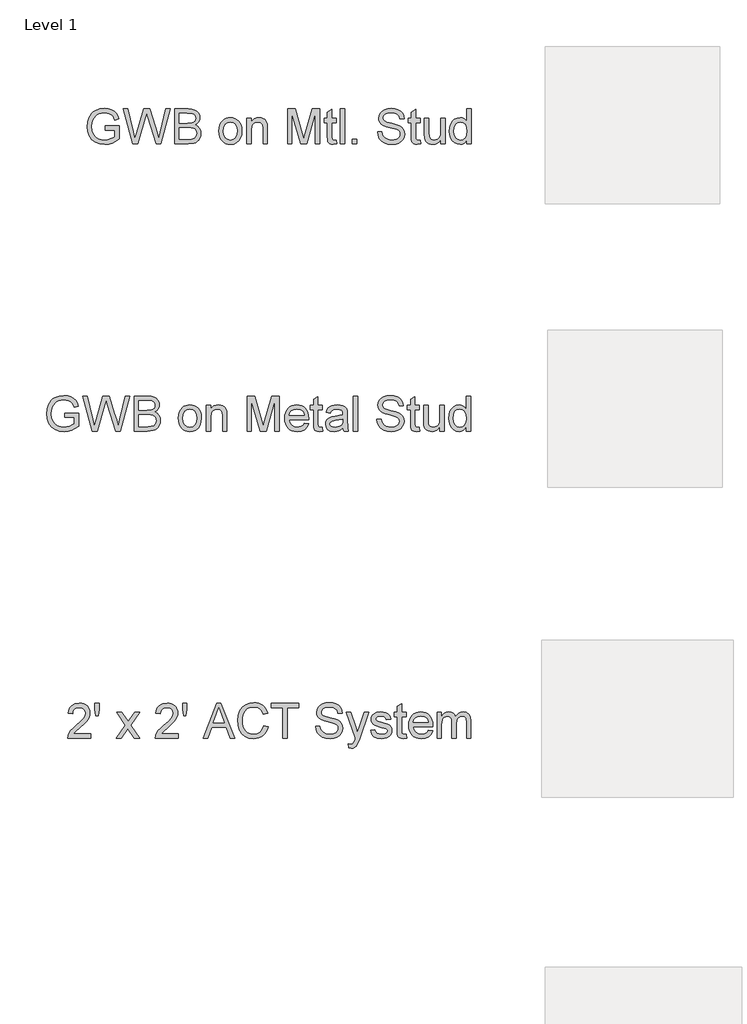
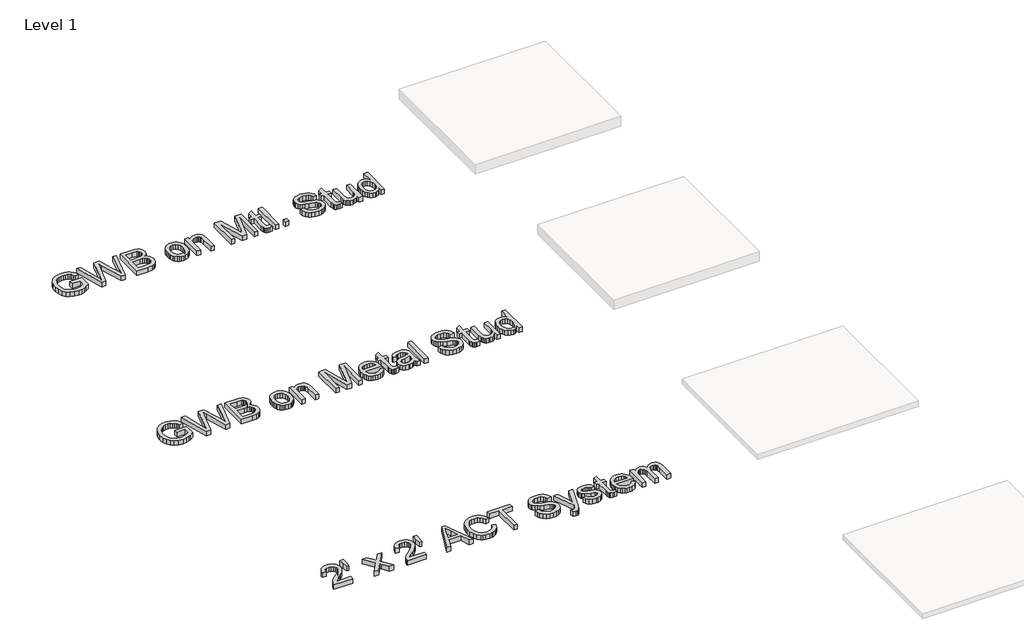
# One storey, part 11 of 42: 3 proxies.
"""IFC4 building model written with IfcOpenShell, lengths in millimetres."""

from ifc_helpers import new_model, si_unit, origin, origin_with_axes, place, context, project, spatial, polyline, outline, extrude, element, save

model = new_model("IFC4")

# Units and contexts
model_context = context("Model", 3, world=origin())
ifc_project = project(units=[si_unit("LENGTHUNIT", "METRE", prefix="MILLI")], contexts=[model_context])

# Site, building, storey
site = spatial("IfcSite", under=ifc_project)
building = spatial("IfcBuilding", under=site)
storey = spatial("IfcBuildingStorey", under=building, Name="Level 1", Elevation=0.0)

# Proxies
placement = place(None, origin())
element("IfcBuildingElementProxy", 1, Name="8\" Arial", ObjectType="8\" Arial", at=placement, inside=storey, context=model_context, shape_type="SweptSolid", body=[
    extrude(outline(polyline([(6999.2760884, -8581.268146), (6999.2760884, -8543.1972592), (7123.0064704, -8543.1972592), (7123.0064704, -8657.0381335), (7092.9382773, -8677.9510962), (7061.92203, -8692.9526615), (7030.0320856, -8701.9870613), (6997.3428012, -8704.998528), (6954.633884, -8700.2117832), (6916.0332022, -8685.8515488), (6883.9666594, -8662.4197359), (6860.8601593, -8630.4182557), (6846.8903002, -8592.0313508), (6842.2336805, -8549.4432641), (6846.8717109, -8506.5484539), (6860.7858021, -8466.6465211), (6883.3996858, -8433.1764862), (6897.7529492, -8420.1430631), (6914.1370936, -8409.5773696), (6951.5759442, -8395.5796266), (6994.294156, -8390.9137122), (7025.6543054, -8393.6184554), (7053.8542737, -8401.7326849), (7077.6021047, -8414.6708378), (7095.6058419, -8431.8473512), (7108.9250755, -8454.0894489), (7118.6193955, -8482.2243547), (7083.5227968, -8492.1138624), (7075.6874068, -8472.0467128), (7066.1603904, -8456.9057278), (7053.5568449, -8445.4918975), (7036.4918674, -8436.606212), (7016.1458783, -8430.8900022), (6993.6992984, -8428.984599), (6967.4233226, -8431.0387166), (6944.9581533, -8437.2010696), (6926.3874424, -8446.700202), (6911.7948418, -8458.7646578), (6892.2017194, -8488.0985735), (6883.2788553, -8516.8376316), (6880.3045673, -8547.8817629), (6883.8830076, -8584.2889073), (6894.6183284, -8614.2455645), (6912.1852171, -8637.5379576), (6936.2583608, -8653.9523097), (6964.4304452, -8663.6838083), (6994.294156, -8666.9276412), (7020.6630783, -8664.4831482), (7046.3813751, -8657.1496693), (7068.7164192, -8647.0463847), (7084.9355836, -8636.2924745), (7084.9355836, -8581.268146), (6999.2760884, -8581.268146)])), origin_with_axes(), (0.0, 0.0, 1.0), 50.8),
    extrude(outline(polyline([(7239.3754895, -8700.2396671), (7156.3184963, -8395.6725731), (7195.5790983, -8395.6725731), (7243.7625643, -8595.8421573), (7258.6340045, -8657.6329911), (7274.5464454, -8602.9804486), (7334.9244924, -8395.6725731), (7391.5103221, -8395.6725731), (7435.3810705, -8545.9484757), (7454.174853, -8601.7163762), (7468.0238816, -8657.6329911), (7482.4491786, -8597.6267302), (7531.0787878, -8395.6725731), (7570.3393898, -8395.6725731), (7487.2080394, -8700.2396671), (7446.5346506, -8700.2396671), (7373.5158795, -8465.2709129), (7363.328943, -8432.4793874), (7351.8779341, -8471.963061), (7285.3282395, -8700.2396671), (7239.3754895, -8700.2396671)])), origin_with_axes(), (0.0, 0.0, 1.0), 50.8),
    extrude(outline(polyline([(7608.4102766, -8700.2396671), (7608.4102766, -8395.6725731), (7724.6305812, -8395.6725731), (7756.5948829, -8397.9125837), (7781.5510184, -8404.6326157), (7800.6794083, -8415.9999728), (7815.1604731, -8432.1819586), (7824.2785248, -8451.217402), (7827.3178754, -8471.1451318), (7824.7618466, -8489.4834764), (7817.0937603, -8506.7250523), (7804.2578485, -8521.8102694), (7786.1983434, -8533.6795376), (7807.7712263, -8544.9446535), (7823.7115512, -8562.0839882), (7833.5545856, -8583.9635945), (7836.8355971, -8609.4495251), (7834.5955864, -8630.6878005), (7827.8755544, -8650.3831641), (7817.846627, -8667.1321235), (7805.67993, -8679.5311867), (7790.7806059, -8688.5098187), (7772.5537971, -8694.9974845), (7723.7382948, -8700.2396671), (7608.4102766, -8700.2396671)]), holes=[polyline([(7646.4811633, -8519.402955), (7716.005146, -8519.402955), (7756.6041775, -8516.1312382), (7770.8156975, -8510.4893856), (7781.030518, -8502.0405487), (7787.192871, -8490.9148525), (7789.2469887, -8477.2424222), (7787.3322907, -8463.9696619), (7781.588197, -8452.4071172), (7772.2749576, -8443.382012), (7759.6528228, -8437.7215701), (7710.7257847, -8433.7434598), (7646.4811633, -8433.7434598), (7646.4811633, -8519.402955)]), polyline([(7646.4811633, -8662.1687804), (7724.556224, -8662.1687804), (7752.8119603, -8660.6816364), (7776.7178003, -8652.3908085), (7792.5558841, -8635.4745453), (7797.2125038, -8623.5216253), (7798.7647103, -8609.8213111), (7796.9429589, -8593.9088701), (7791.4777047, -8580.2271452), (7781.932099, -8569.5290029), (7767.8692935, -8562.56731), (7747.9508583, -8558.7472088), (7720.838364, -8557.4738418), (7646.4811633, -8557.4738418), (7646.4811633, -8662.1687804)])]), origin_with_axes(), (0.0, 0.0, 1.0), 50.8),
    extrude(outline(polyline([(7993.878005, -8588.4064373), (7995.93677, -8559.4396603), (8002.113065, -8534.4788775), (8012.4068899, -8513.5240888), (8026.8182449, -8496.5752944), (8041.3271937, -8485.7423797), (8057.3418758, -8478.0045835), (8074.8622912, -8473.3619058), (8093.8884399, -8471.8143466), (8114.8920255, -8473.6988369), (8133.8833193, -8479.3523078), (8150.8623213, -8488.7747593), (8165.8290316, -8501.9661915), (8178.0445255, -8518.480461), (8186.7698782, -8537.8714247), (8192.0050899, -8560.1390827), (8193.7501605, -8585.2834348), (8190.6643366, -8623.7446969), (8181.4068651, -8653.0228447), (8166.2472909, -8674.9489242), (8145.4551586, -8691.3539816), (8120.7592733, -8701.5873914), (8093.8884399, -8704.998528), (8072.5781309, -8703.1210087), (8053.4102388, -8697.4884507), (8036.3847635, -8688.1008541), (8021.501705, -8674.9582189), (8009.4163363, -8658.2836166), (8000.78393, -8638.3001189), (7995.6044862, -8615.0077258), (7993.878005, -8588.4064373)]), holes=[polyline([(8031.9488917, -8588.3320801), (8036.3545559, -8622.7873479), (8049.5715483, -8647.3345188), (8069.4620995, -8662.0293606), (8093.8884399, -8666.9276412), (8118.2032446, -8662.0014767), (8138.0566171, -8647.222983), (8151.2736096, -8622.3504994), (8155.6792737, -8587.1423649), (8151.2457256, -8553.6909192), (8137.9450813, -8529.4783557), (8118.0638248, -8514.7835139), (8093.8884399, -8509.8852333), (8069.4620995, -8514.7649246), (8049.5715483, -8529.4039985), (8036.3545559, -8553.8954015), (8031.9488917, -8588.3320801)])]), origin_with_axes(), (0.0, 0.0, 1.0), 50.8),
    extrude(outline(polyline([(8236.5799081, -8700.2396671), (8236.5799081, -8476.5732074), (8274.6507948, -8476.5732074), (8274.6507948, -8507.8032317), (8287.8770819, -8492.0580945), (8303.7616389, -8480.8115679), (8322.3044658, -8474.0636519), (8343.5055627, -8471.8143466), (8362.2714612, -8473.6268033), (8379.4572692, -8479.0641736), (8393.7896196, -8487.447948), (8403.9951454, -8498.099617), (8415.4089758, -8526.0951031), (8417.4166202, -8562.9019174), (8417.4166202, -8700.2396671), (8379.3457334, -8700.2396671), (8379.3457334, -8568.0325643), (8374.9586586, -8534.3487524), (8368.8892521, -8524.3198249), (8359.4551822, -8516.5402028), (8347.3628425, -8511.5489757), (8333.3186262, -8509.8852333), (8311.0207606, -8513.6216827), (8292.0132012, -8524.8310307), (8284.4171484, -8533.9816137), (8278.9913964, -8546.4875654), (8274.6507948, -8581.5655748), (8274.6507948, -8700.2396671), (8236.5799081, -8700.2396671)])), origin_with_axes(), (0.0, 0.0, 1.0), 50.8),
    extrude(outline(polyline([(8593.4944714, -8700.2396671), (8593.4944714, -8395.6725731), (8659.0031652, -8395.6725731), (8721.3144994, -8610.3418115), (8733.8808664, -8655.1792035), (8747.4882341, -8606.6239514), (8808.7585675, -8395.6725731), (8874.2672613, -8395.6725731), (8874.2672613, -8700.2396671), (8836.1963745, -8700.2396671), (8836.1963745, -8433.7434598), (8759.682815, -8700.2396671), (8708.0789177, -8700.2396671), (8631.5653582, -8433.7434598), (8631.5653582, -8700.2396671), (8593.4944714, -8700.2396671)])), origin_with_axes(), (0.0, 0.0, 1.0), 50.8),
    extrude(outline(polyline([(9017.0330866, -8668.4891424), (9021.7919475, -8701.3550251), (8993.3131396, -8704.998528), (8975.0398575, -8703.4184375), (8961.4139005, -8698.6781659), (8951.784643, -8691.3725709), (8945.5014595, -8682.0965102), (8942.0438497, -8666.1654799), (8940.8913131, -8638.8949765), (8940.8913131, -8514.6440942), (8912.338148, -8514.6440942), (8912.338148, -8476.5732074), (8940.8913131, -8476.5732074), (8940.8913131, -8422.2180937), (8978.9621999, -8399.8365763), (8978.9621999, -8476.5732074), (9017.0330866, -8476.5732074), (9017.0330866, -8514.6440942), (8978.9621999, -8514.6440942), (8978.9621999, -8637.7796185), (8980.9698443, -8657.4099195), (8987.4760993, -8664.3623178), (9000.4514309, -8666.9276412), (9017.0330866, -8668.4891424)])), origin_with_axes(), (0.0, 0.0, 1.0), 50.8),
    extrude(outline(polyline([(9055.1039734, -8700.2396671), (9055.1039734, -8395.6725731), (9093.1748601, -8395.6725731), (9093.1748601, -8700.2396671), (9055.1039734, -8700.2396671)])), origin_with_axes(), (0.0, 0.0, 1.0), 50.8),
    extrude(outline(polyline([(9159.798912, -8700.2396671), (9159.798912, -8662.1687804), (9197.8697987, -8662.1687804), (9197.8697987, -8700.2396671), (9159.798912, -8700.2396671)])), origin_with_axes(), (0.0, 0.0, 1.0), 50.8),
    extrude(outline(polyline([(9378.7065108, -8595.5447285), (9416.7773976, -8595.5447285), (9421.1458831, -8616.6714682), (9429.0463357, -8633.6527939), (9441.3710417, -8647.1300365), (9459.0122876, -8657.7445269), (9480.5758758, -8664.6318626), (9504.6676088, -8666.9276412), (9525.8780003, -8665.1895416), (9544.4487112, -8659.9752429), (9559.4967497, -8651.7215937), (9570.139124, -8640.8654424), (9576.4687807, -8628.4013166), (9578.5786663, -8615.3237439), (9576.9985758, -8602.5807787), (9572.2583042, -8591.5666183), (9562.6290468, -8582.1697271), (9546.3819984, -8574.2785691), (9490.9487053, -8559.7417364), (9454.5601502, -8550.1217736), (9431.2770517, -8540.9665432), (9412.3252602, -8528.1585154), (9398.8944908, -8512.6364498), (9390.8917971, -8494.7349537), (9388.2242325, -8474.7886346), (9391.5238333, -8452.490769), (9401.4226356, -8431.6986368), (9417.6603893, -8414.0759802), (9439.9768442, -8401.2865417), (9466.7640258, -8393.5069196), (9496.4139595, -8390.9137122), (9528.5362702, -8393.62775), (9556.6432921, -8401.7698635), (9579.7312029, -8415.1727489), (9596.7961805, -8433.6691026), (9607.5965639, -8456.1063879), (9611.8906922, -8481.3320683), (9573.8198055, -8481.3320683), (9566.8302286, -8458.6159434), (9552.2562173, -8442.2201807), (9529.4843245, -8432.2934944), (9497.9011035, -8428.984599), (9465.5743105, -8432.2563158), (9443.3972754, -8442.0714663), (9430.5706583, -8456.5153525), (9426.2951193, -8473.6732766), (9429.3251752, -8488.3030558), (9438.415343, -8500.0700828), (9459.904574, -8510.5916267), (9500.5779628, -8521.3362422), (9542.5526026, -8531.541768), (9567.9455866, -8540.4460428), (9589.6485946, -8554.2578928), (9604.7895796, -8571.3042811), (9613.6845597, -8591.3993146), (9616.6495531, -8614.3571003), (9613.2384165, -8637.8260918), (9603.0050067, -8659.9008857), (9586.3675831, -8678.8991505), (9563.7444048, -8693.1385545), (9536.538964, -8702.0335346), (9506.1547528, -8704.998528), (9468.855322, -8701.8011683), (9438.1550928, -8692.2090894), (9413.7008684, -8676.1851127), (9395.1394522, -8653.6920595), (9383.2237108, -8626.291431), (9378.7065108, -8595.5447285)])), origin_with_axes(), (0.0, 0.0, 1.0), 50.8),
    extrude(outline(polyline([(9749.8976567, -8668.4891424), (9754.6565176, -8701.3550251), (9726.1777097, -8704.998528), (9707.9044276, -8703.4184375), (9694.2784706, -8698.6781659), (9684.6492131, -8691.3725709), (9678.3660296, -8682.0965102), (9674.9084198, -8666.1654799), (9673.7558832, -8638.8949765), (9673.7558832, -8514.6440942), (9645.2027181, -8514.6440942), (9645.2027181, -8476.5732074), (9673.7558832, -8476.5732074), (9673.7558832, -8422.2180937), (9711.82677, -8399.8365763), (9711.82677, -8476.5732074), (9749.8976567, -8476.5732074), (9749.8976567, -8514.6440942), (9711.82677, -8514.6440942), (9711.82677, -8637.7796185), (9713.8344144, -8657.4099195), (9720.3406694, -8664.3623178), (9733.316001, -8666.9276412), (9749.8976567, -8668.4891424)])), origin_with_axes(), (0.0, 0.0, 1.0), 50.8),
    extrude(outline(polyline([(9930.7343688, -8700.2396671), (9930.7343688, -8661.7969944), (9916.9596974, -8680.6976653), (9900.9171313, -8694.1981446), (9882.6066707, -8702.2984321), (9862.0283154, -8704.998528), (9843.4854885, -8703.1024194), (9826.2253232, -8697.4140935), (9811.7442584, -8688.8630154), (9801.5387326, -8678.3786501), (9794.6699862, -8665.6449795), (9790.1992595, -8650.3459855), (9787.9685435, -8614.9519579), (9787.9685435, -8476.5732074), (9826.0394302, -8476.5732074), (9826.0394302, -8597.0318726), (9828.3445035, -8635.8463313), (9833.8934096, -8648.7937789), (9843.4018366, -8658.6368133), (9856.2377484, -8664.8549342), (9871.7691087, -8666.9276412), (9888.1927554, -8664.808461), (9903.556812, -8658.4509203), (9916.22542, -8648.4405822), (9924.5627212, -8635.3630095), (9929.1914569, -8617.4522188), (9930.7343688, -8592.9422265), (9930.7343688, -8476.5732074), (9968.8052556, -8476.5732074), (9968.8052556, -8700.2396671), (9930.7343688, -8700.2396671)])), origin_with_axes(), (0.0, 0.0, 1.0), 50.8),
    extrude(outline(polyline([(10159.1596894, -8700.2396671), (10159.1596894, -8664.3251392), (10147.7690957, -8682.1197468), (10133.9711876, -8694.8301808), (10117.7659652, -8702.4564412), (10099.1534284, -8704.998528), (10074.541195, -8701.3178465), (10052.0109632, -8690.2758022), (10032.9383412, -8672.643851), (10018.6989373, -8649.1934488), (10009.8318411, -8620.87265), (10006.8761423, -8588.6295089), (10009.5994748, -8556.7860377), (10017.7694722, -8528.0283903), (10031.37684, -8503.9924252), (10050.4122834, -8486.3140007), (10073.4351316, -8475.4392601), (10099.004714, -8471.8143466), (10117.6311928, -8474.4075539), (10134.1013127, -8482.1871761), (10148.0618772, -8494.1122121), (10159.1596894, -8509.1416613), (10159.1596894, -8395.6725731), (10197.2305761, -8395.6725731), (10197.2305761, -8700.2396671), (10159.1596894, -8700.2396671)]), holes=[polyline([(10044.9470291, -8588.4807945), (10049.2411574, -8622.917473), (10062.1235425, -8647.408876), (10080.8429677, -8662.0479499), (10102.6482168, -8666.9276412), (10124.4441713, -8662.2710215), (10142.6895694, -8648.3011624), (10155.0421594, -8624.7578138), (10159.1596894, -8591.3807253), (10154.9678022, -8554.8899291), (10142.3921406, -8529.5898915), (10123.68201, -8514.8113979), (10101.0867156, -8509.8852333), (10079.0583949, -8514.6162102), (10061.0081845, -8528.8091409), (10048.9623179, -8553.1890081), (10044.9470291, -8588.4807945)])]), origin_with_axes(), (0.0, 0.0, 1.0), 50.8),
])
element("IfcBuildingElementProxy", 2, Name="8\" Arial", ObjectType="8\" Arial", at=placement, inside=storey, context=model_context, shape_type="SweptSolid", body=[
    extrude(outline(polyline([(6872.0666272, -13851.3846733), (6872.0666272, -13889.45556), (6672.1944717, -13889.45556), (6676.2841177, -13863.2074682), (6685.6717143, -13842.6941754), (6699.4092072, -13822.7943296), (6719.281169, -13801.9650187), (6747.0721728, -13778.663331), (6788.1545262, -13742.1725347), (6812.8039382, -13715.2366388), (6825.1286442, -13693.3756218), (6829.2368796, -13672.1094624), (6825.3610105, -13653.046135), (6813.7334032, -13637.1987566), (6795.8597911, -13626.5192037), (6773.2459074, -13622.9593527), (6749.4980765, -13626.4355518), (6731.0481961, -13636.8641492), (6719.1417493, -13653.4272157), (6715.0242193, -13675.306822), (6676.9533325, -13670.5479612), (6680.227373, -13650.8944235), (6686.1829201, -13633.7225575), (6694.8199737, -13619.032363), (6706.1385338, -13606.8238402), (6719.8783503, -13597.2271139), (6735.7791729, -13590.3723095), (6774.0638367, -13584.888466), (6794.4679173, -13586.4127886), (6812.6273399, -13590.9857564), (6828.5421045, -13598.6073695), (6842.2122111, -13609.2776278), (6853.1915165, -13622.2064861), (6861.0338775, -13636.603899), (6865.7392941, -13652.4698667), (6867.3077663, -13669.8043892), (6865.61614, -13688.0126087), (6860.5412611, -13705.9048101), (6851.5347451, -13724.103735), (6838.0482079, -13743.2321248), (6816.5496822, -13766.0690801), (6783.5072011, -13795.3937011), (6739.7108099, -13832.0146225), (6722.5342966, -13851.3846733), (6872.0666272, -13851.3846733)])), origin_with_axes(), (0.0, 0.0, 1.0), 50.8),
    extrude(outline(polyline([(6918.688592, -13694.3422654), (6910.1375139, -13636.5667204), (6910.1375139, -13584.888466), (6948.2084007, -13584.888466), (6948.2084007, -13636.5667204), (6939.2855366, -13694.3422654), (6918.688592, -13694.3422654)])), origin_with_axes(), (0.0, 0.0, 1.0), 50.8),
    extrude(outline(polyline([(7095.7330869, -13889.45556), (7177.0798645, -13777.0274726), (7100.4919477, -13665.7891003), (7146.2959834, -13665.7891003), (7183.2515121, -13719.3262848), (7200.5023827, -13744.6077331), (7215.44818, -13723.9364313), (7257.5343556, -13665.7891003), (7303.3383912, -13665.7891003), (7222.8839001, -13777.0274726), (7300.3641032, -13889.45556), (7254.5600676, -13889.45556), (7207.9381027, -13821.8648646), (7199.3870247, -13809.5215693), (7141.5371225, -13889.45556), (7095.7330869, -13889.45556)])), origin_with_axes(), (0.0, 0.0, 1.0), 50.8),
    extrude(outline(polyline([(7638.2432232, -13851.3846733), (7638.2432232, -13889.45556), (7438.3710677, -13889.45556), (7442.4607138, -13863.2074682), (7451.8483103, -13842.6941754), (7465.5858032, -13822.7943296), (7485.4577651, -13801.9650187), (7513.2487688, -13778.663331), (7554.3311222, -13742.1725347), (7578.9805342, -13715.2366388), (7591.3052403, -13693.3756218), (7595.4134756, -13672.1094624), (7591.5376065, -13653.046135), (7579.9099992, -13637.1987566), (7562.0363871, -13626.5192037), (7539.4225035, -13622.9593527), (7515.6746725, -13626.4355518), (7497.2247921, -13636.8641492), (7485.3183453, -13653.4272157), (7481.2008153, -13675.306822), (7443.1299286, -13670.5479612), (7446.4039691, -13650.8944235), (7452.3595161, -13633.7225575), (7460.9965697, -13619.032363), (7472.3151298, -13606.8238402), (7486.0549463, -13597.2271139), (7501.955769, -13590.3723095), (7540.2404327, -13584.888466), (7560.6445133, -13586.4127886), (7578.8039359, -13590.9857564), (7594.7187005, -13598.6073695), (7608.3888071, -13609.2776278), (7619.3681125, -13622.2064861), (7627.2104735, -13636.603899), (7631.9158901, -13652.4698667), (7633.4843623, -13669.8043892), (7631.792736, -13688.0126087), (7626.7178571, -13705.9048101), (7617.7113412, -13724.103735), (7604.2248039, -13743.2321248), (7582.7262782, -13766.0690801), (7549.6837972, -13795.3937011), (7505.8874059, -13832.0146225), (7488.7108926, -13851.3846733), (7638.2432232, -13851.3846733)])), origin_with_axes(), (0.0, 0.0, 1.0), 50.8),
    extrude(outline(polyline([(7684.865188, -13694.3422654), (7676.31411, -13636.5667204), (7676.31411, -13584.888466), (7714.3849967, -13584.888466), (7714.3849967, -13636.5667204), (7705.4621326, -13694.3422654), (7684.865188, -13694.3422654)])), origin_with_axes(), (0.0, 0.0, 1.0), 50.8),
    extrude(outline(polyline([(7854.9944632, -13889.45556), (7976.5684864, -13584.888466), (8008.9882259, -13584.888466), (8130.562249, -13889.45556), (8090.3350035, -13889.45556), (8055.4614763, -13794.2783431), (7930.0208787, -13794.2783431), (7895.2217088, -13889.45556), (7854.9944632, -13889.45556)]), holes=[polyline([(7944.0000325, -13756.2074564), (8041.5566798, -13756.2074564), (8014.1188727, -13681.3297553), (7992.7783561, -13622.9593527), (7973.81727, -13674.7863216), (7944.0000325, -13756.2074564)])]), origin_with_axes(), (0.0, 0.0, 1.0), 50.8),
    extrude(outline(polyline([(8385.3843758, -13781.1914758), (8423.4552626, -13791.0066263), (8415.9219487, -13814.6824237), (8405.8883739, -13835.3699912), (8393.3545383, -13853.0693286), (8378.3204418, -13867.780436), (8361.1253391, -13879.3453044), (8342.108485, -13887.6059247), (8321.2698795, -13892.5622968), (8298.6095226, -13894.2144209), (8254.45064, -13889.2138991), (8235.7800117, -13882.9632469), (8219.3819253, -13874.2123339), (8192.5017972, -13849.7302255), (8172.9086748, -13816.2880745), (8160.9464602, -13776.9717047), (8156.9590553, -13734.8669398), (8161.4669606, -13690.4571016), (8174.9906764, -13652.1073754), (8196.8238095, -13621.0353601), (8226.2599663, -13598.4586551), (8261.1706721, -13584.7118676), (8299.4274518, -13580.1296051), (8321.2024933, -13581.6121018), (8341.1697254, -13586.0595919), (8359.329148, -13593.4720753), (8375.6807611, -13603.8495521), (8389.95502, -13616.9178302), (8401.8823797, -13632.4027172), (8418.6964017, -13670.6223184), (8380.625515, -13679.6938968), (8367.4271119, -13651.930777), (8349.3954907, -13632.886039), (8326.3075799, -13621.8718787), (8297.9403078, -13618.2004919), (8265.2417288, -13622.2715486), (8238.38019, -13634.4847188), (8217.9970224, -13653.5573408), (8204.7335567, -13678.2067528), (8197.4558457, -13706.0721138), (8195.029942, -13734.7925826), (8197.9019889, -13769.9635385), (8206.5181295, -13800.3756336), (8221.2036767, -13824.8670366), (8242.2839431, -13842.2759162), (8267.5560967, -13852.6766296), (8294.8173054, -13856.1435341), (8326.595714, -13851.4218519), (8353.0761721, -13837.2568051), (8373.0689645, -13813.7971083), (8385.3843758, -13781.1914758)])), origin_with_axes(), (0.0, 0.0, 1.0), 50.8),
    extrude(outline(polyline([(8551.9445054, -13889.45556), (8551.9445054, -13622.9593527), (8452.0084277, -13622.9593527), (8452.0084277, -13584.888466), (8689.9514699, -13584.888466), (8689.9514699, -13622.9593527), (8590.0153922, -13622.9593527), (8590.0153922, -13889.45556), (8551.9445054, -13889.45556)])), origin_with_axes(), (0.0, 0.0, 1.0), 50.8),
    extrude(outline(polyline([(8837.4761561, -13784.7606214), (8875.5470428, -13784.7606214), (8879.9155284, -13805.8873611), (8887.815981, -13822.8686868), (8900.140687, -13836.3459294), (8917.7819328, -13846.9604198), (8939.345521, -13853.8477555), (8963.4372541, -13856.1435341), (8984.6476456, -13854.4054345), (9003.2183564, -13849.1911358), (9018.2663949, -13840.9374866), (9028.9087693, -13830.0813353), (9035.238426, -13817.6172095), (9037.3483116, -13804.5396368), (9035.7682211, -13791.7966716), (9031.0279495, -13780.7825112), (9021.398692, -13771.38562), (9005.1516437, -13763.494462), (8949.7183505, -13748.9576293), (8913.3297955, -13739.3376665), (8890.046697, -13730.1824361), (8871.0949055, -13717.3744083), (8857.6641361, -13701.8523427), (8849.6614424, -13683.9508466), (8846.9938778, -13664.0045275), (8850.2934786, -13641.7066619), (8860.1922809, -13620.9145297), (8876.4300346, -13603.2918731), (8898.7464895, -13590.5024346), (8925.533671, -13582.7228125), (8955.1836048, -13580.1296051), (8987.3059155, -13582.8436429), (9015.4129374, -13590.9857564), (9038.5008482, -13604.3886418), (9055.5658257, -13622.8849955), (9066.3662091, -13645.3222808), (9070.6603375, -13670.5479612), (9032.5894507, -13670.5479612), (9025.5998739, -13647.8318363), (9011.0258625, -13631.4360736), (8988.2539698, -13621.5093873), (8956.6707488, -13618.2004919), (8924.3439558, -13621.4722087), (8902.1669207, -13631.2873592), (8889.3403036, -13645.7312454), (8885.0647645, -13662.8891695), (8888.0948205, -13677.5189487), (8897.1849883, -13689.2859757), (8918.6742193, -13699.8075196), (8959.347608, -13710.5521351), (9001.3222478, -13720.7576609), (9026.7152319, -13729.6619357), (9048.4182398, -13743.4737857), (9063.5592248, -13760.520174), (9072.454205, -13780.6152075), (9075.4191983, -13803.5729932), (9072.0080617, -13827.0419847), (9061.774652, -13849.1167786), (9045.1372283, -13868.1150434), (9022.51405, -13882.3544474), (8995.3086092, -13891.2494275), (8964.9243981, -13894.2144209), (8927.6249673, -13891.0170612), (8896.924738, -13881.4249823), (8872.4705137, -13865.4010056), (8853.9090974, -13842.9079524), (8841.993356, -13815.5073239), (8837.4761561, -13784.7606214)])), origin_with_axes(), (0.0, 0.0, 1.0), 50.8),
    extrude(outline(polyline([(9127.7666676, -13975.1150552), (9123.0078068, -13938.4569553), (9142.340679, -13941.8030293), (9160.4094787, -13937.6018475), (9171.4887016, -13925.8905884), (9181.8987097, -13897.8579237), (9184.8729978, -13888.6376308), (9103.9723634, -13665.7891003), (9144.1252518, -13665.7891003), (9187.0293566, -13789.9656255), (9201.9751539, -13839.6362356), (9216.9209513, -13795.7654871), (9261.0147713, -13665.7891003), (9300.8702309, -13665.7891003), (9223.0182417, -13894.8092785), (9202.7930831, -13944.4798885), (9192.4388429, -13960.3365616), (9180.7089945, -13971.322838), (9167.0830375, -13977.7361466), (9151.0404714, -13979.8739161), (9127.7666676, -13975.1150552)])), origin_with_axes(), (0.0, 0.0, 1.0), 50.8),
    extrude(outline(polyline([(9318.1211014, -13822.8315082), (9356.1919882, -13818.0726473), (9362.1963321, -13834.3568743), (9373.8146447, -13846.3283836), (9391.1212832, -13853.6897465), (9414.1906047, -13856.1435341), (9436.9810867, -13853.8942288), (9453.0050635, -13847.1463128), (9462.4856066, -13837.3683409), (9465.6457876, -13826.0288678), (9462.4670173, -13816.3252531), (9452.9307063, -13808.9267117), (9413.7444615, -13798.0705604), (9356.4150598, -13779.4440816), (9341.906111, -13770.0843689), (9331.3938617, -13757.6946004), (9325.0084371, -13743.0648211), (9322.8799623, -13726.9850765), (9324.5901779, -13712.2344668), (9329.7208247, -13698.6178044), (9337.8071703, -13686.6741791), (9348.3844821, -13676.9426804), (9372.5877509, -13665.6775645), (9405.3420978, -13661.0302395), (9430.121635, -13662.8984641), (9451.6666339, -13668.5031381), (9468.9918616, -13677.2958771), (9481.1120854, -13688.7282967), (9489.142663, -13703.6462101), (9494.1989527, -13722.8954305), (9456.1280659, -13727.6542913), (9451.3227318, -13715.6734873), (9441.8143048, -13706.6483821), (9427.5098383, -13700.9879402), (9408.3163859, -13699.1011262), (9386.4553689, -13700.9042883), (9371.8813575, -13706.3137747), (9363.6834761, -13714.1212808), (9360.950849, -13723.1185021), (9365.4866383, -13734.197725), (9379.6888636, -13742.6000886), (9412.4803891, -13750.7050235), (9468.3598254, -13768.6251089), (9483.1197298, -13777.1947763), (9494.3104885, -13788.9246247), (9501.3651279, -13803.8518327), (9503.7166744, -13822.013579), (9500.9561633, -13840.7887722), (9492.6746301, -13858.4486073), (9479.1880928, -13873.6081816), (9460.8125696, -13884.8825922), (9438.6169451, -13891.8814637), (9413.6701043, -13894.2144209), (9375.2831995, -13889.7158102), (9347.2691241, -13876.2199783), (9328.5682881, -13853.8756395), (9318.1211014, -13822.8315082)])), origin_with_axes(), (0.0, 0.0, 1.0), 50.8),
    extrude(outline(polyline([(9627.4470563, -13857.7050353), (9632.2059172, -13890.570918), (9603.7271093, -13894.2144209), (9585.4538272, -13892.6343304), (9571.8278702, -13887.8940588), (9562.1986127, -13880.5884638), (9555.9154293, -13871.3124031), (9552.4578194, -13855.3813728), (9551.3052828, -13828.1108694), (9551.3052828, -13703.8599871), (9522.7521177, -13703.8599871), (9522.7521177, -13665.7891003), (9551.3052828, -13665.7891003), (9551.3052828, -13611.4339866), (9589.3761696, -13589.0524692), (9589.3761696, -13665.7891003), (9627.4470563, -13665.7891003), (9627.4470563, -13703.8599871), (9589.3761696, -13703.8599871), (9589.3761696, -13826.9955114), (9591.383814, -13846.6258124), (9597.890069, -13853.5782107), (9610.8654006, -13856.1435341), (9627.4470563, -13857.7050353)])), origin_with_axes(), (0.0, 0.0, 1.0), 50.8),
    extrude(outline(polyline([(9822.1142078, -13822.8315082), (9859.4415225, -13827.590369), (9845.9921638, -13855.7159802), (9824.5308168, -13876.7404787), (9795.5408032, -13889.8459353), (9759.5054448, -13894.2144209), (9735.8830916, -13892.3299306), (9714.8353565, -13886.6764596), (9696.3622394, -13877.2540081), (9680.4637404, -13864.062576), (9667.6789492, -13847.4693019), (9658.5469555, -13827.8413246), (9653.0677593, -13805.178644), (9651.2413606, -13779.4812602), (9653.0863486, -13752.9125029), (9658.6213127, -13729.494632), (9667.8462529, -13709.2276475), (9680.7611692, -13692.1115494), (9696.6178423, -13678.5134763), (9714.6680527, -13668.8005669), (9734.9118006, -13662.9728213), (9757.349086, -13661.0302395), (9779.0637122, -13662.968174), (9798.7009842, -13668.7819776), (9816.2609019, -13678.4716504), (9831.7434653, -13692.0371922), (9844.3818657, -13709.1161117), (9853.4092946, -13729.3459176), (9858.8257519, -13752.7266099), (9860.6312377, -13779.2581886), (9860.4081661, -13789.5194823), (9689.3122473, -13789.5194823), (9695.9021542, -13818.0168794), (9711.2104429, -13838.9670207), (9733.3038262, -13851.8494058), (9760.2490168, -13856.1435341), (9780.511354, -13854.154479), (9797.5763315, -13848.1873136), (9811.4439495, -13837.870252), (9822.1142078, -13822.8315082)]), holes=[polyline([(9689.3122473, -13751.4485955), (9822.560351, -13751.4485955), (9817.4111148, -13731.3349727), (9807.3171248, -13716.9468544), (9785.1215004, -13703.5625583), (9757.2003716, -13699.1011262), (9731.5378427, -13702.6609772), (9710.3181565, -13713.3405302), (9695.5675468, -13729.9872485), (9689.3122473, -13751.4485955)])]), origin_with_axes(), (0.0, 0.0, 1.0), 50.8),
    extrude(outline(polyline([(9898.7021245, -13889.45556), (9898.7021245, -13665.7891003), (9936.7730112, -13665.7891003), (9936.7730112, -13702.5959147), (9948.2240201, -13685.6889462), (9962.9467459, -13672.4440698), (9980.4392774, -13663.883697), (10000.1997034, -13661.0302395), (10021.3729163, -13663.9394649), (10038.3449474, -13672.6671414), (10051.0228501, -13686.6370005), (10059.313678, -13705.2727739), (10073.1905906, -13685.9166651), (10089.0193797, -13672.0908731), (10106.8000453, -13663.7953979), (10126.5325874, -13661.0302395), (10155.150815, -13665.6310913), (10176.3147333, -13679.4336466), (10189.392306, -13702.8096916), (10193.7514969, -13736.1310122), (10193.7514969, -13889.45556), (10155.6806101, -13889.45556), (10155.6806101, -13752.4895963), (10152.1486431, -13720.701893), (10147.1852999, -13711.937038), (10139.3592045, -13705.0497023), (10129.2930985, -13700.5882702), (10117.6097233, -13699.1011262), (10096.9848948, -13702.9119328), (10080.1708728, -13714.3443524), (10068.9894087, -13734.1791357), (10065.2622541, -13763.1970332), (10065.2622541, -13889.45556), (10027.1913673, -13889.45556), (10027.1913673, -13748.2512359), (10024.9885352, -13726.7248263), (10018.380039, -13711.3700643), (10006.7524318, -13702.1683608), (9989.4922665, -13699.1011262), (9974.8253087, -13701.1459492), (9961.3108875, -13707.2804183), (9950.1573074, -13717.355819), (9942.5728729, -13731.2234369), (9938.2229767, -13750.4633626), (9936.7730112, -13776.6556866), (9936.7730112, -13889.45556), (9898.7021245, -13889.45556)])), origin_with_axes(), (0.0, 0.0, 1.0), 50.8),
])
element("IfcBuildingElementProxy", 3, Name="8\" Arial", ObjectType="8\" Arial", at=placement, inside=storey, context=model_context, shape_type="SweptSolid", body=[
    extrude(outline(polyline([(6645.1845795, -11089.0835074), (6645.1845795, -11051.0126206), (6768.9149614, -11051.0126206), (6768.9149614, -11164.8534949), (6738.8467684, -11185.7664576), (6707.8305211, -11200.7680228), (6675.9405766, -11209.8024227), (6643.2512923, -11212.8138893), (6600.5423751, -11208.0271445), (6561.9416933, -11193.6669101), (6529.8751505, -11170.2350973), (6506.7686504, -11138.233617), (6492.7987913, -11099.8467122), (6488.1421716, -11057.2586255), (6492.780202, -11014.3638153), (6506.6942932, -10974.4618825), (6529.3081768, -10940.9918475), (6543.6614402, -10927.9584244), (6560.0455847, -10917.3927309), (6597.4844352, -10903.3949879), (6640.202647, -10898.7290736), (6671.5627964, -10901.4338167), (6699.7627648, -10909.5480463), (6723.5105958, -10922.4861992), (6741.514333, -10939.6627126), (6754.8335666, -10961.9048102), (6764.5278866, -10990.039716), (6729.4312879, -10999.9292237), (6721.5958978, -10979.8620742), (6712.0688815, -10964.7210892), (6699.465336, -10953.3072589), (6682.4003584, -10944.4215734), (6662.0543694, -10938.7053636), (6639.6077894, -10936.7999603), (6613.3318136, -10938.854078), (6590.8666444, -10945.016431), (6572.2959335, -10954.5155634), (6557.7033329, -10966.5800192), (6538.1102105, -10995.9139349), (6529.1873464, -11024.652993), (6526.2130584, -11055.6971242), (6529.7914986, -11092.1042686), (6540.5268195, -11122.0609259), (6558.0937082, -11145.353319), (6582.1668519, -11161.767671), (6610.3389363, -11171.4991697), (6640.202647, -11174.7430026), (6666.5715693, -11172.2985096), (6692.2898661, -11164.9650307), (6714.6249103, -11154.861746), (6730.8440747, -11144.1078359), (6730.8440747, -11089.0835074), (6645.1845795, -11089.0835074)])), origin_with_axes(), (0.0, 0.0, 1.0), 50.8),
    extrude(outline(polyline([(6885.2839805, -11208.0550285), (6802.2269874, -10903.4879344), (6841.4875893, -10903.4879344), (6889.6710554, -11103.6575187), (6904.5424955, -11165.4483525), (6920.4549365, -11110.79581), (6980.8329834, -10903.4879344), (7037.4188132, -10903.4879344), (7081.2895616, -11053.763837), (7100.0833441, -11109.5317375), (7113.9323727, -11165.4483525), (7128.3576696, -11105.4420915), (7176.9872789, -10903.4879344), (7216.2478809, -10903.4879344), (7133.1165305, -11208.0550285), (7092.4431417, -11208.0550285), (7019.4243706, -10973.0862743), (7009.2374341, -10940.2947488), (6997.7864252, -10979.7784223), (6931.2367306, -11208.0550285), (6885.2839805, -11208.0550285)])), origin_with_axes(), (0.0, 0.0, 1.0), 50.8),
    extrude(outline(polyline([(7254.3187676, -11208.0550285), (7254.3187676, -10903.4879344), (7370.5390723, -10903.4879344), (7402.503374, -10905.7279451), (7427.4595094, -10912.4479771), (7446.5878993, -10923.8153342), (7461.0689642, -10939.99732), (7470.1870159, -10959.0327633), (7473.2263665, -10978.9604931), (7470.6703377, -10997.2988377), (7463.0022514, -11014.5404137), (7450.1663396, -11029.6256307), (7432.1068345, -11041.4948989), (7453.6797173, -11052.7600148), (7469.6200422, -11069.8993496), (7479.4630767, -11091.7789559), (7482.7440882, -11117.2648864), (7480.5040775, -11138.5031619), (7473.7840455, -11158.1985254), (7463.755118, -11174.9474849), (7451.5884211, -11187.3465481), (7436.689097, -11196.3251801), (7418.4622882, -11202.8128458), (7369.6467859, -11208.0550285), (7254.3187676, -11208.0550285)]), holes=[polyline([(7292.3896544, -11027.2183164), (7361.913637, -11027.2183164), (7402.5126686, -11023.9465995), (7416.7241886, -11018.3047469), (7426.939009, -11009.85591), (7433.101362, -10998.7302139), (7435.1554797, -10985.0577836), (7433.2407818, -10971.7850233), (7427.496688, -10960.2224785), (7418.1834487, -10951.1973733), (7405.5613138, -10945.5369314), (7356.6342758, -10941.5588212), (7292.3896544, -10941.5588212), (7292.3896544, -11027.2183164)]), polyline([(7292.3896544, -11169.9841417), (7370.4647151, -11169.9841417), (7398.7204514, -11168.4969977), (7422.6262914, -11160.2061698), (7438.4643751, -11143.2899067), (7443.1209948, -11131.3369867), (7444.6732014, -11117.6366724), (7442.85145, -11101.7242315), (7437.3861957, -11088.0425065), (7427.8405901, -11077.3443643), (7413.7777845, -11070.3826714), (7393.8593494, -11066.5625702), (7366.7468551, -11065.2892031), (7292.3896544, -11065.2892031), (7292.3896544, -11169.9841417)])]), origin_with_axes(), (0.0, 0.0, 1.0), 50.8),
    extrude(outline(polyline([(7639.786496, -11096.2217986), (7641.845261, -11067.2550216), (7648.021556, -11042.2942388), (7658.315381, -11021.3394502), (7672.726736, -11004.3906558), (7687.2356847, -10993.5577411), (7703.2503668, -10985.8199449), (7720.7707823, -10981.1772672), (7739.796931, -10979.6297079), (7760.8005165, -10981.5141982), (7779.7918103, -10987.1676691), (7796.7708124, -10996.5901207), (7811.7375227, -11009.7815528), (7823.9530165, -11026.2958224), (7832.6783693, -11045.6867861), (7837.913581, -11067.954444), (7839.6586515, -11093.0987962), (7836.5728277, -11131.5600583), (7827.3153562, -11160.838206), (7812.1557819, -11182.7642856), (7791.3636497, -11199.169343), (7766.6677644, -11209.4027527), (7739.796931, -11212.8138893), (7718.486622, -11210.93637), (7699.3187299, -11205.3038121), (7682.2932546, -11195.9162155), (7667.4101961, -11182.7735802), (7655.3248273, -11166.098978), (7646.6924211, -11146.1154803), (7641.5129773, -11122.8230872), (7639.786496, -11096.2217986)]), holes=[polyline([(7677.8573828, -11096.1474414), (7682.2630469, -11130.6027093), (7695.4800394, -11155.1498802), (7715.3705906, -11169.844722), (7739.796931, -11174.7430026), (7764.1117356, -11169.816838), (7783.9651082, -11155.0383444), (7797.1821006, -11130.1658607), (7801.5877648, -11094.9577262), (7797.1542167, -11061.5062805), (7783.8535724, -11037.2937171), (7763.9723159, -11022.5988753), (7739.796931, -11017.7005947), (7715.3705906, -11022.580286), (7695.4800394, -11037.2193599), (7682.2630469, -11061.7107628), (7677.8573828, -11096.1474414)])]), origin_with_axes(), (0.0, 0.0, 1.0), 50.8),
    extrude(outline(polyline([(7882.4883991, -11208.0550285), (7882.4883991, -10984.3885688), (7920.5592859, -10984.3885688), (7920.5592859, -11015.6185931), (7933.785573, -10999.8734558), (7949.67013, -10988.6269292), (7968.2129569, -10981.8790132), (7989.4140537, -10979.6297079), (8008.1799523, -10981.4421647), (8025.3657603, -10986.879535), (8039.6981107, -10995.2633094), (8049.9036365, -11005.9149784), (8061.3174668, -11033.9104644), (8063.3251112, -11070.7172788), (8063.3251112, -11208.0550285), (8025.2542245, -11208.0550285), (8025.2542245, -11075.8479256), (8020.8671496, -11042.1641137), (8014.7977431, -11032.1351863), (8005.3636733, -11024.3555641), (7993.2713335, -11019.3643371), (7979.2271172, -11017.7005947), (7956.9292517, -11021.437044), (7937.9216922, -11032.646392), (7930.3256395, -11041.796975), (7924.8998875, -11054.3029267), (7920.5592859, -11089.3809362), (7920.5592859, -11208.0550285), (7882.4883991, -11208.0550285)])), origin_with_axes(), (0.0, 0.0, 1.0), 50.8),
    extrude(outline(polyline([(8239.4029625, -11208.0550285), (8239.4029625, -10903.4879344), (8304.9116563, -10903.4879344), (8367.2229905, -11118.1571728), (8379.7893574, -11162.9945649), (8393.3967251, -11114.4393128), (8454.6670585, -10903.4879344), (8520.1757523, -10903.4879344), (8520.1757523, -11208.0550285), (8482.1048656, -11208.0550285), (8482.1048656, -10941.5588212), (8405.5913061, -11208.0550285), (8353.9874088, -11208.0550285), (8277.4738492, -10941.5588212), (8277.4738492, -11208.0550285), (8239.4029625, -11208.0550285)])), origin_with_axes(), (0.0, 0.0, 1.0), 50.8),
    extrude(outline(polyline([(8738.637208, -11141.4309767), (8775.9645227, -11146.1898375), (8762.5151641, -11174.3154487), (8741.053817, -11195.3399472), (8712.0638034, -11208.4454038), (8676.028445, -11212.8138893), (8652.4060918, -11210.929399), (8631.3583567, -11205.2759281), (8612.8852396, -11195.8534766), (8596.9867407, -11182.6620444), (8584.2019495, -11166.0687704), (8575.0699558, -11146.440793), (8569.5907595, -11123.7781125), (8567.7643608, -11098.0807286), (8569.6093488, -11071.5119714), (8575.144313, -11048.0941005), (8584.3692532, -11027.827116), (8597.2841695, -11010.7110178), (8613.1408425, -10997.1129447), (8631.191053, -10987.4000354), (8651.4348009, -10981.5722898), (8673.8720862, -10979.6297079), (8695.5867124, -10981.5676425), (8715.2239844, -10987.3814461), (8732.7839021, -10997.0711188), (8748.2664655, -11010.6366606), (8760.9048659, -11027.7155802), (8769.9322948, -11047.9453861), (8775.3487522, -11071.3260784), (8777.154238, -11097.857657), (8776.9311664, -11108.1189507), (8605.8352475, -11108.1189507), (8612.4251545, -11136.6163479), (8627.7334431, -11157.5664892), (8649.8268264, -11170.4488742), (8676.772017, -11174.7430026), (8697.0343542, -11172.7539474), (8714.0993318, -11166.7867821), (8727.9669497, -11156.4697205), (8738.637208, -11141.4309767)]), holes=[polyline([(8605.8352475, -11070.048064), (8739.0833512, -11070.048064), (8733.934115, -11049.9344412), (8723.8401251, -11035.5463229), (8701.6445006, -11022.1620267), (8673.7233718, -11017.7005947), (8648.0608429, -11021.2604457), (8626.8411567, -11031.9399986), (8612.090547, -11048.5867169), (8605.8352475, -11070.048064)])]), origin_with_axes(), (0.0, 0.0, 1.0), 50.8),
    extrude(outline(polyline([(8896.1257591, -11176.3045038), (8900.8846199, -11209.1703865), (8872.4058121, -11212.8138893), (8854.13253, -11211.2337988), (8840.506573, -11206.4935273), (8830.8773155, -11199.1879323), (8824.594132, -11189.9118715), (8821.1365222, -11173.9808413), (8819.9839856, -11146.7103379), (8819.9839856, -11022.4594555), (8791.4308205, -11022.4594555), (8791.4308205, -10984.3885688), (8819.9839856, -10984.3885688), (8819.9839856, -10930.0334551), (8858.0548723, -10907.6519376), (8858.0548723, -10984.3885688), (8896.1257591, -10984.3885688), (8896.1257591, -11022.4594555), (8858.0548723, -11022.4594555), (8858.0548723, -11145.5949799), (8860.0625167, -11165.2252809), (8866.5687718, -11172.1776791), (8879.5441033, -11174.7430026), (8896.1257591, -11176.3045038)])), origin_with_axes(), (0.0, 0.0, 1.0), 50.8),
    extrude(outline(polyline([(9076.9624712, -11179.5018634), (9058.772841, -11195.0982863), (9040.044121, -11205.3038121), (9020.3487575, -11210.93637), (8999.2591964, -11212.8138893), (8967.4436092, -11208.2966894), (8943.9746177, -11194.7450896), (8929.5028475, -11174.1667343), (8924.6789241, -11148.5692679), (8926.5006756, -11132.7869521), (8931.9659298, -11118.4546016), (8940.3961774, -11106.1856635), (8951.112909, -11096.5935846), (8977.7699654, -11084.1015749), (9010.7102054, -11078.3760705), (9049.6361999, -11072.3531372), (9076.7393996, -11065.2892031), (9076.9624712, -11056.8124823), (9074.3413799, -11039.8218619), (9066.4781059, -11028.7054604), (9048.8926279, -11020.4518111), (9024.3919303, -11017.7005947), (9001.7129841, -11019.5316408), (8985.8749003, -11025.024779), (8975.0745169, -11035.1838315), (8967.5086717, -11051.0126206), (8929.437785, -11046.2537598), (8936.0462812, -11025.4337436), (8945.9079049, -11009.0751594), (8959.9428266, -10996.5645604), (8979.0712165, -10987.2884996), (9002.4658507, -10981.5444058), (9029.2995055, -10979.6297079), (9055.0363916, -10981.3213342), (9075.4381486, -10986.3962132), (9090.8207945, -10994.0271209), (9101.5003474, -11003.3868336), (9108.5828708, -11014.9586729), (9113.1744279, -11029.2259608), (9115.0333579, -11062.5379867), (9115.0333579, -11109.9035236), (9116.9666452, -11176.0442536), (9124.5510796, -11208.0550285), (9086.4801929, -11208.0550285), (9080.3829024, -11194.8194468), (9076.9624712, -11179.5018634)]), holes=[polyline([(9076.9624712, -11103.3600899), (9015.5434234, -11115.0341704), (8982.7890765, -11121.2058181), (8967.954815, -11131.2440402), (8962.7498109, -11145.8924087), (8965.5846792, -11157.2132925), (8974.089284, -11166.4893533), (8988.0777324, -11172.6795902), (9007.3641313, -11174.7430026), (9027.8123615, -11172.4658133), (9045.8811613, -11165.6342455), (9060.5295298, -11155.5681394), (9070.7164663, -11143.5873355), (9075.2336663, -11131.2440402), (9076.7393996, -11114.141884), (9076.9624712, -11103.3600899)])]), origin_with_axes(), (0.0, 0.0, 1.0), 50.8),
    extrude(outline(polyline([(9167.3808272, -11208.0550285), (9167.3808272, -10903.4879344), (9205.451714, -10903.4879344), (9205.451714, -11208.0550285), (9167.3808272, -11208.0550285)])), origin_with_axes(), (0.0, 0.0, 1.0), 50.8),
    extrude(outline(polyline([(9372.0118436, -11103.3600899), (9410.0827303, -11103.3600899), (9414.4512159, -11124.4868295), (9422.3516684, -11141.4681553), (9434.6763744, -11154.9453979), (9452.3176203, -11165.5598883), (9473.8812085, -11172.447224), (9497.9729415, -11174.7430026), (9519.183333, -11173.004903), (9537.7540439, -11167.7906043), (9552.8020824, -11159.536955), (9563.4444568, -11148.6808037), (9569.7741135, -11136.216678), (9571.883999, -11123.1391053), (9570.3039085, -11110.39614), (9565.563637, -11099.3819797), (9555.9343795, -11089.9850884), (9539.6873311, -11082.0939305), (9484.254038, -11067.5570978), (9447.8654829, -11057.9371349), (9424.5823845, -11048.7819046), (9405.6305929, -11035.9738768), (9392.1998235, -11020.4518111), (9384.1971298, -11002.550315), (9381.5295652, -10982.603996), (9384.829166, -10960.3061304), (9394.7279684, -10939.5139981), (9410.9657221, -10921.8913416), (9433.2821769, -10909.1019031), (9460.0693585, -10901.3222809), (9489.7192923, -10898.7290736), (9521.841603, -10901.4431114), (9549.9486248, -10909.5852249), (9573.0365356, -10922.9881103), (9590.1015132, -10941.484464), (9600.9018966, -10963.9217493), (9605.196025, -10989.1474296), (9567.1251382, -10989.1474296), (9560.1355613, -10966.4313048), (9545.56155, -10950.035542), (9522.7896573, -10940.1088558), (9491.2064363, -10936.7999603), (9458.8796433, -10940.0716772), (9436.7026082, -10949.8868276), (9423.875991, -10964.3307139), (9419.600452, -10981.4886379), (9422.6305079, -10996.1184172), (9431.7206757, -11007.8854442), (9453.2099067, -11018.4069881), (9493.8832955, -11029.1516036), (9535.8579353, -11039.3571294), (9561.2509193, -11048.2614042), (9582.9539273, -11062.0732542), (9598.0949123, -11079.1196425), (9606.9898924, -11099.214676), (9609.9548858, -11122.1724617), (9606.5437492, -11145.6414531), (9596.3103395, -11167.7162471), (9579.6729158, -11186.7145119), (9557.0497375, -11200.9539158), (9529.8442967, -11209.8488959), (9499.4600856, -11212.8138893), (9462.1606548, -11209.6165297), (9431.4604255, -11200.0244508), (9407.0062011, -11184.0004741), (9388.4447849, -11161.5074208), (9376.5290435, -11134.1067924), (9372.0118436, -11103.3600899)])), origin_with_axes(), (0.0, 0.0, 1.0), 50.8),
    extrude(outline(polyline([(9743.2029895, -11176.3045038), (9747.9618503, -11209.1703865), (9719.4830424, -11212.8138893), (9701.2097604, -11211.2337988), (9687.5838033, -11206.4935273), (9677.9545458, -11199.1879323), (9671.6713624, -11189.9118715), (9668.2137525, -11173.9808413), (9667.0612159, -11146.7103379), (9667.0612159, -11022.4594555), (9638.5080509, -11022.4594555), (9638.5080509, -10984.3885688), (9667.0612159, -10984.3885688), (9667.0612159, -10930.0334551), (9705.1321027, -10907.6519376), (9705.1321027, -10984.3885688), (9743.2029895, -10984.3885688), (9743.2029895, -11022.4594555), (9705.1321027, -11022.4594555), (9705.1321027, -11145.5949799), (9707.1397471, -11165.2252809), (9713.6460022, -11172.1776791), (9726.6213337, -11174.7430026), (9743.2029895, -11176.3045038)])), origin_with_axes(), (0.0, 0.0, 1.0), 50.8),
    extrude(outline(polyline([(9924.0397016, -11208.0550285), (9924.0397016, -11169.6123557), (9910.2650301, -11188.5130267), (9894.2224641, -11202.0135059), (9875.9120034, -11210.1137935), (9855.3336481, -11212.8138893), (9836.7908212, -11210.9177807), (9819.530656, -11205.2294549), (9805.0495911, -11196.6783768), (9794.8440653, -11186.1940115), (9787.9753189, -11173.4603409), (9783.5045922, -11158.1613468), (9781.2738762, -11122.7673193), (9781.2738762, -10984.3885688), (9819.344763, -10984.3885688), (9819.344763, -11104.8472339), (9821.6498362, -11143.6616927), (9827.1987423, -11156.6091402), (9836.7071693, -11166.4521747), (9849.5430811, -11172.6702956), (9865.0744414, -11174.7430026), (9881.4980881, -11172.6238223), (9896.8621447, -11166.2662817), (9909.5307528, -11156.2559435), (9917.8680539, -11143.1783709), (9922.4967896, -11125.2675801), (9924.0397016, -11100.7575879), (9924.0397016, -10984.3885688), (9962.1105883, -10984.3885688), (9962.1105883, -11208.0550285), (9924.0397016, -11208.0550285)])), origin_with_axes(), (0.0, 0.0, 1.0), 50.8),
    extrude(outline(polyline([(10152.4650221, -11208.0550285), (10152.4650221, -11172.1405005), (10141.0744284, -11189.9351081), (10127.2765204, -11202.6455421), (10111.0712979, -11210.2718025), (10092.4587611, -11212.8138893), (10067.8465277, -11209.1332079), (10045.3162959, -11198.0911636), (10026.2436739, -11180.4592124), (10012.00427, -11157.0088102), (10003.1371738, -11128.6880114), (10000.1814751, -11096.4448702), (10002.9048075, -11064.601399), (10011.074805, -11035.8437517), (10024.6821727, -11011.8077865), (10043.7176161, -10994.1293621), (10066.7404643, -10983.2546215), (10092.3100467, -10979.6297079), (10110.9365255, -10982.2229153), (10127.4066455, -10990.0025374), (10141.3672099, -11001.9275735), (10152.4650221, -11016.9570227), (10152.4650221, -10903.4879344), (10190.5359089, -10903.4879344), (10190.5359089, -11208.0550285), (10152.4650221, -11208.0550285)]), holes=[polyline([(10038.2523618, -11096.2961558), (10042.5464902, -11130.7328344), (10055.4288752, -11155.2242374), (10074.1483005, -11169.8633113), (10095.9535496, -11174.7430026), (10117.749504, -11170.0863829), (10135.9949022, -11156.1165238), (10148.3474921, -11132.5731751), (10152.4650221, -11099.1960867), (10148.2731349, -11062.7052904), (10135.6974733, -11037.4052529), (10116.9873427, -11022.6267592), (10094.3920484, -11017.7005947), (10072.3637277, -11022.4315716), (10054.3135172, -11036.6245023), (10042.2676507, -11061.0043694), (10038.2523618, -11096.2961558)])]), origin_with_axes(), (0.0, 0.0, 1.0), 50.8),
])

save(model, "model.ifc")

# Revit data of these elements
# Elements 1, 2, 3 (IfcBuildingElementProxy, "8\" Arial")
#   Phase Created = New Construction
